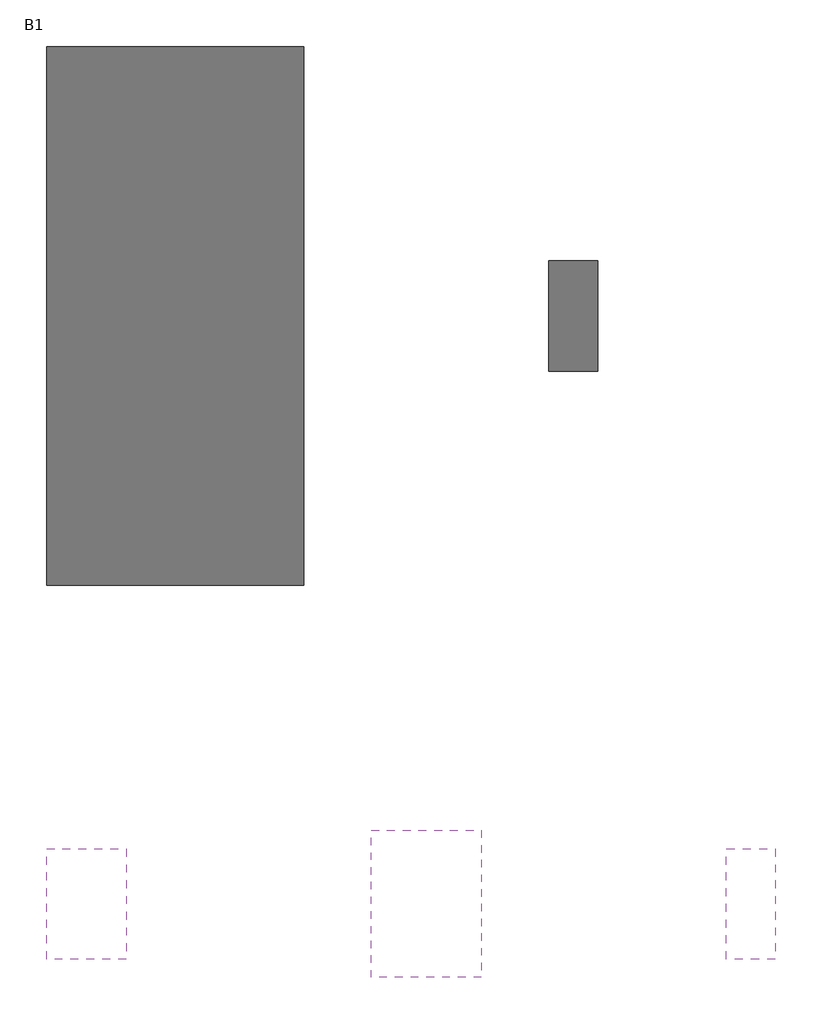
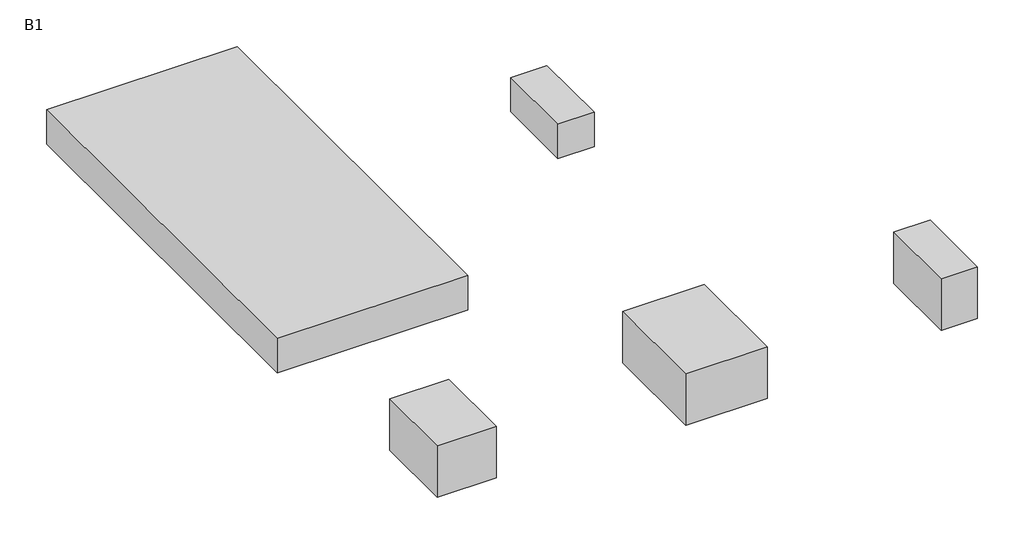
# One storey: 5 proxies.
"""IFC4 building model written with IfcOpenShell, lengths in millimetres."""

import ifcopenshell
import ifcopenshell.guid

model = None  # the IFC model being written
_history = None  # IfcOwnerHistory: only IFC2X3 demands one
_inside = {}  # id of a spatial element -> (the spatial element, [elements in it])
_under = {}  # id of a project, library or spatial element -> (it, [spatial elements below it])
_declared = {}  # id of a project -> (the project, [libraries it declares])
_typed = {}  # id of a type object -> (the type object, [elements of that type])
_made_of = {}  # id of a material, layer set ... -> (it, [elements and type objects made of it])


def new_model(schema):
    """Start an empty IFC model of exactly this schema.

    Asked for "IFC4X3", IfcOpenShell would pick the latest addendum, in which some entities
    have other attributes; the version numbers below select the first issue.
    IFC2X3 requires an IfcOwnerHistory on every rooted entity: one is made here for all.
    """
    global model, _history
    if schema == "IFC4X3":
        model = ifcopenshell.file(schema_version=(4, 3, 0, 0))
    else:
        model = ifcopenshell.file(schema=schema)
    _inside.clear()
    _under.clear()
    _declared.clear()
    _typed.clear()
    _made_of.clear()
    _history = None
    if model.schema == "IFC2X3":
        org = make("IfcOrganization", Name="unknown")
        user = make(
            "IfcPersonAndOrganization",
            ThePerson=make("IfcPerson", FamilyName="unknown"),
            TheOrganization=org,
        )
        app = make(
            "IfcApplication",
            ApplicationDeveloper=org,
            Version="unknown",
            ApplicationFullName="unknown",
            ApplicationIdentifier="unknown",
        )
        _history = make(
            "IfcOwnerHistory",
            OwningUser=user,
            OwningApplication=app,
            ChangeAction="ADDED",
            CreationDate=0,
        )
    return model


def make(cls, **values):
    """One entity of the class cls with the attributes given. An attribute that is None is left unset."""
    return model.create_entity(
        cls, **{name: value for name, value in values.items() if value is not None}
    )


def rooted(cls, **values):
    """An entity with a GlobalId (a new one), such as an element, a storey or a relation."""
    return make(cls, GlobalId=ifcopenshell.guid.new(), OwnerHistory=_history, **values)


def si_unit(unit_type, name, prefix=None):
    """IfcSIUnit, for example si_unit("LENGTHUNIT", "METRE", prefix="MILLI")."""
    return make("IfcSIUnit", UnitType=unit_type, Prefix=prefix, Name=name)


def assignment(units):
    """IfcUnitAssignment: the units of a project."""
    return None if units is None else make("IfcUnitAssignment", Units=units)


def point(xyz):
    """IfcCartesianPoint."""
    return None if xyz is None else make("IfcCartesianPoint", Coordinates=xyz)


def direction(xyz):
    """IfcDirection."""
    return None if xyz is None else make("IfcDirection", DirectionRatios=xyz)


def frame(location, z_axis=None, x_axis=None):
    """IfcAxis2Placement3D, a coordinate frame: its origin and axes. An axis left out is left unset."""
    return make(
        "IfcAxis2Placement3D",
        Location=point(location),
        Axis=direction(z_axis),
        RefDirection=direction(x_axis),
    )


def origin():
    """The frame at (0, 0, 0) with its axes left unset."""
    return frame((0.0, 0.0, 0.0))


def origin_with_axes():
    """The frame at (0, 0, 0) with the z axis (0, 0, 1) and the x axis (1, 0, 0) written out."""
    return frame((0.0, 0.0, 0.0), z_axis=(0.0, 0.0, 1.0), x_axis=(1.0, 0.0, 0.0))


def place(relative_to, where):
    """IfcLocalPlacement: puts the frame where relative to a parent placement (None: the world)."""
    return make(
        "IfcLocalPlacement", PlacementRelTo=relative_to, RelativePlacement=where
    )


def context(
    kind, dimensions, precision=None, world=None, true_north=None, identifier=None
):
    """IfcGeometricRepresentationContext, for example the 3D "Model" context."""
    return make(
        "IfcGeometricRepresentationContext",
        ContextIdentifier=identifier,
        ContextType=kind,
        CoordinateSpaceDimension=dimensions,
        Precision=precision,
        WorldCoordinateSystem=world,
        TrueNorth=true_north,
    )


def project(units=None, contexts=None):
    """IfcProject with its units and contexts."""
    return rooted(
        "IfcProject",
        Name="project",
        RepresentationContexts=contexts,
        UnitsInContext=assignment(units),
    )


def spatial(cls, under=None, at=None, **own):
    """A site, building, storey or space (cls), placed at a placement, below another one or the project."""
    s = rooted(cls, ObjectPlacement=at, **own)
    if under is not None:
        _under.setdefault(under.id(), (under, []))[1].append(s)
    return s


def polyline(points):
    """IfcPolyline through the points."""
    return make("IfcPolyline", Points=[point(p) for p in points])


def outline(outer, holes=None, kind="AREA"):
    """IfcArbitraryClosedProfileDef: a profile drawn as a closed curve; with holes, ...WithVoids."""
    if holes is None:
        return make("IfcArbitraryClosedProfileDef", ProfileType=kind, OuterCurve=outer)
    return make(
        "IfcArbitraryProfileDefWithVoids",
        ProfileType=kind,
        OuterCurve=outer,
        InnerCurves=holes,
    )


def extrude(swept, where, along, depth):
    """IfcExtrudedAreaSolid: the profile swept, set in the frame where, extruded along a direction by depth."""
    return make(
        "IfcExtrudedAreaSolid",
        SweptArea=swept,
        Position=where,
        ExtrudedDirection=direction(along),
        Depth=depth,
    )


def shape(context_of_items, identifier, shape_type, items):
    """IfcShapeRepresentation: the items that make up one representation, for example the "Body"."""
    return make(
        "IfcShapeRepresentation",
        ContextOfItems=context_of_items,
        RepresentationIdentifier=identifier,
        RepresentationType=shape_type,
        Items=items,
    )


def source(mapping_origin, context_of_items, identifier, shape_type, items):
    """IfcRepresentationMap: a shape defined once, which mapped items show again and again."""
    return make(
        "IfcRepresentationMap",
        MappingOrigin=mapping_origin,
        MappedRepresentation=shape(context_of_items, identifier, shape_type, items),
    )


def transform(
    local_origin,
    x_axis=None,
    y_axis=None,
    z_axis=None,
    scale=None,
    scale2=None,
    scale3=None,
    uniform=True,
):
    """IfcCartesianTransformationOperator3D, or its non-uniform kind. x_axis, y_axis, z_axis: its Axis1, 2, 3."""
    if uniform:
        return make(
            "IfcCartesianTransformationOperator3D",
            Axis1=direction(x_axis),
            Axis2=direction(y_axis),
            LocalOrigin=point(local_origin),
            Scale=scale,
            Axis3=direction(z_axis),
        )
    return make(
        "IfcCartesianTransformationOperator3DnonUniform",
        Axis1=direction(x_axis),
        Axis2=direction(y_axis),
        LocalOrigin=point(local_origin),
        Scale=scale,
        Axis3=direction(z_axis),
        Scale2=scale2,
        Scale3=scale3,
    )


def mapped(mapping_source, mapping_target):
    """IfcMappedItem: shows the shape of a source again, moved by a transform."""
    return make(
        "IfcMappedItem", MappingSource=mapping_source, MappingTarget=mapping_target
    )


def made_of(thing, what):
    """Note that an element or type object is made of a material, layer set ...; save() writes the relation."""
    if what is not None:
        _made_of.setdefault(what.id(), (what, []))[1].append(thing)
    return thing


def element(
    cls,
    number,
    at=None,
    inside=None,
    cuts=None,
    type_object=None,
    material=None,
    context=None,
    identifier="Body",
    shape_type=None,
    held_by="IfcProductDefinitionShape",
    body=None,
    shapes=None,
    **own,
):
    """One element of the class cls, such as IfcWall. Its Tag is "e" and its number.

    at: its placement. inside: the storey or other place that contains it. cuts: it is an
    opening in that element (IfcRelVoidsElement). A single representation is given by context,
    identifier, shape_type and body (its items); several are given by shapes. held_by: the class
    of the entity that holds the representations. save() writes the other relations.
    """
    e = rooted(cls, Tag="e%d" % number, ObjectPlacement=at, **own)
    if body is not None:
        shapes = [shape(context, identifier, shape_type, body)]
    if shapes is not None:
        e.Representation = make(held_by, Representations=shapes)
    if inside is not None:
        _inside.setdefault(inside.id(), (inside, []))[1].append(e)
    if cuts is not None:
        rooted(
            "IfcRelVoidsElement", RelatingBuildingElement=cuts, RelatedOpeningElement=e
        )
    if type_object is not None:
        _typed.setdefault(type_object.id(), (type_object, []))[1].append(e)
    return made_of(e, material)


def aggregate(whole, parts):
    """IfcRelAggregates: a whole, such as a stair, and the parts it consists of."""
    return rooted("IfcRelAggregates", RelatingObject=whole, RelatedObjects=parts)


def save(model, path):
    """Write the relations noted so far, then the file.

    IfcRelAggregates (storeys below a building ...), IfcRelContainedInSpatialStructure (elements
    in a storey), IfcRelDefinesByType, IfcRelAssociatesMaterial and IfcRelDeclares: one each for
    every whole, place, type object, material and project.
    """
    for whole, parts in _under.values():
        aggregate(whole, parts)
    for where, things in _inside.values():
        rooted(
            "IfcRelContainedInSpatialStructure",
            RelatedElements=things,
            RelatingStructure=where,
        )
    for kind, things in _typed.values():
        rooted("IfcRelDefinesByType", RelatedObjects=things, RelatingType=kind)
    for what, things in _made_of.values():
        rooted("IfcRelAssociatesMaterial", RelatedObjects=things, RelatingMaterial=what)
    for by, libraries in _declared.values():
        rooted("IfcRelDeclares", RelatingContext=by, RelatedDefinitions=libraries)
    model.write(path)


def generic_models_1d705098(model_context):
    return source(origin(), model_context, "Body", "SweptSolid", [
        extrude(outline(polyline([(3250.0, 4500.0), (3250.0, -4500.0), (-3250.0, -4500.0), (-3250.0, 4500.0), (3250.0, 4500.0)])), origin_with_axes(), (0.0, 0.0, 1.0), 6000.0),
    ])


def generic_models_399a6151(model_context):
    return source(origin(), model_context, "Body", "SweptSolid", [
        extrude(outline(polyline([(4500.0, 6000.0), (4500.0, -6000.0), (-4500.0, -6000.0), (-4500.0, 6000.0), (4500.0, 6000.0)])), origin_with_axes(), (0.0, 0.0, 1.0), 6000.0),
    ])


def generic_models_29bcd6f9(model_context):
    return source(origin(), model_context, "Body", "SweptSolid", [
        extrude(outline(polyline([(2000.0, 4500.0), (2000.0, -4500.0), (-2000.0, -4500.0), (-2000.0, 4500.0), (2000.0, 4500.0)])), origin_with_axes(), (0.0, 0.0, 1.0), 6000.0),
    ])


def generic_models_a454a2aa(model_context):
    return source(origin(), model_context, "Body", "SweptSolid", [
        extrude(outline(polyline([(10500.0, 22000.0), (10500.0, -22000.0), (-10500.0, -22000.0), (-10500.0, 22000.0), (10500.0, 22000.0)])), origin_with_axes(), (0.0, 0.0, 1.0), 4000.0),
    ])


def generic_models_73802227(model_context):
    return source(origin(), model_context, "Body", "SweptSolid", [
        extrude(outline(polyline([(2000.0, 4500.0), (2000.0, -4500.0), (-2000.0, -4500.0), (-2000.0, 4500.0), (2000.0, 4500.0)])), origin_with_axes(), (0.0, 0.0, 1.0), 4000.0),
    ])


model = new_model("IFC4")

# Units and contexts
model_context = context("Model", 3, world=origin())
ifc_project = project(units=[si_unit("LENGTHUNIT", "METRE", prefix="MILLI")], contexts=[model_context])

# Site, building, storey
site = spatial("IfcSite", under=ifc_project)
building = spatial("IfcBuilding", under=site)
storey = spatial("IfcBuildingStorey", under=building, Name="B1", Elevation=-4000.0)

# Proxies
placement = place(None, origin())
generic_models_shape = generic_models_1d705098(model_context)
element("IfcBuildingElementProxy", 1, Name="Space Planning Box_hec : Space Planning Box_hec", ObjectType="Space Planning Box_hec : Space Planning Box_hec", at=placement, inside=storey, context=model_context, shape_type="MappedRepresentation", body=[
    mapped(generic_models_shape, transform((3250.0, 6000.0, 0.0), x_axis=(1.0, 0.0, 0.0), y_axis=(0.0, 1.0, 0.0), z_axis=(0.0, 0.0, 1.0))),
])
generic_models_2_shape = generic_models_399a6151(model_context)
element("IfcBuildingElementProxy", 2, Name="Space Planning Box_hec : Space Planning Box_hec", ObjectType="Space Planning Box_hec : Space Planning Box_hec", at=placement, inside=storey, context=model_context, shape_type="MappedRepresentation", body=[
    mapped(generic_models_2_shape, transform((31000.0, 6000.0, 0.0), x_axis=(1.0, 0.0, 0.0), y_axis=(0.0, 1.0, 0.0), z_axis=(0.0, 0.0, 1.0))),
])
generic_models_3_shape = generic_models_29bcd6f9(model_context)
element("IfcBuildingElementProxy", 3, Name="Space Planning Box_hec : Space Planning Box_hec", ObjectType="Space Planning Box_hec : Space Planning Box_hec", at=placement, inside=storey, context=model_context, shape_type="MappedRepresentation", body=[
    mapped(generic_models_3_shape, transform((57500.0, 6000.0, 0.0), x_axis=(1.0, 0.0, 0.0), y_axis=(0.0, 1.0, 0.0), z_axis=(0.0, 0.0, 1.0))),
])
generic_models_4_shape = generic_models_a454a2aa(model_context)
element("IfcBuildingElementProxy", 4, Name="Space Planning Box_hec : Space Planning Box_hec", ObjectType="Space Planning Box_hec : Space Planning Box_hec", at=placement, inside=storey, context=model_context, shape_type="MappedRepresentation", body=[
    mapped(generic_models_4_shape, transform((10500.0, 54000.0, -4000.0), x_axis=(1.0, 0.0, 0.0), y_axis=(0.0, 1.0, 0.0), z_axis=(0.0, 0.0, 1.0))),
])
generic_models_5_shape = generic_models_73802227(model_context)
element("IfcBuildingElementProxy", 5, Name="Space Planning Box_hec : Space Planning Box_hec", ObjectType="Space Planning Box_hec : Space Planning Box_hec", at=placement, inside=storey, context=model_context, shape_type="MappedRepresentation", body=[
    mapped(generic_models_5_shape, transform((43000.0, 54000.0, -4000.0), x_axis=(1.0, 0.0, 0.0), y_axis=(0.0, 1.0, 0.0), z_axis=(0.0, 0.0, 1.0))),
])

save(model, "model.ifc")

# Revit data of these elements
# Project information
#   Building Name = "MAIN GATE SECURITY BUILDING"
#   Project Status = "Project Status"
#   Client Name = "현대엔지니어링"
#   Project Address = "서울시 종로구 율곡로 75(계동)"
#   Project Name = "Therma Visayas Energy Project"
#   Project Number = "-"
# Grids (mm)
#   "A": line (45459.652, 190234.526) -> (45459.652, 152139.384)
#   "B": line (53459.652, 190234.526) -> (53459.652, 152139.384)
#   "C": line (61459.652, 190234.526) -> (61459.652, 152139.384)
#   "D": line (67459.652, 190234.526) -> (67459.652, 152139.384)
#   "E": line (73459.652, 190234.526) -> (73459.652, 152139.384)
#   "F": line (81459.652, 190234.526) -> (81459.652, 152139.384)
#   "G": line (85459.652, 190234.526) -> (85459.652, 152139.384)
#   "H": line (89459.652, 190234.526) -> (89459.652, 152139.384)
#   "4": line (39389.066, 184923.861) -> (102402.798, 184923.861)
#   "3": line (39389.066, 178923.861) -> (102402.798, 178923.861)
#   "2": line (39389.066, 172923.861) -> (102402.798, 172923.861)
#   "1": line (39389.066, 163923.861) -> (102402.798, 163923.861)
# Type "Space Planning Box_hec : Space Planning Box_hec"
#   Type Comments = "..."
#   Room Name [instance default] = "?"
#   Interior Finish [instance default] = ""
#   Exterior Finish [instance default] = ""
#   Department [instance default] = ""
#   Assembly Code = "..."
#   Width [instance default] = 1524 mm
#   Program Area [instance default] = 0.00 m²
#   Length [instance default] = 1524 mm
#   Height [instance default] = 1524 mm
#   Area [instance default] = 2.32258 m²
#   Fill Color [instance default] = Cyan
#   Default Elevation = 0
# Element 1 (IfcBuildingElementProxy, "Space Planning Box_hec : Space Planning Box_hec")
#   Room Name = "Switchgear Room"
#   Interior Finish = "IF1"
#   Exterior Finish = "EF1"
#   Department = "EL"
#   Width = 6500 mm
#   Program Area = 58.50 m²
#   Length = 9000 mm
#   Height = 6000 mm
#   Area = 58.50 m²
#   Fill Color = Blue
#   Phase Created = New Construction
#   Materials on its faces: "Blue"
# Element 2 (IfcBuildingElementProxy, "Space Planning Box_hec : Space Planning Box_hec")
#   Room Name = "Battery Room"
#   Interior Finish = "IF4"
#   Exterior Finish = "EF1"
#   Department = "EL"
#   Width = 9000 mm
#   Program Area = 108.00 m²
#   Length = 12000 mm
#   Height = 6000 mm
#   Area = 108.00 m²
#   Fill Color = Blue
#   Phase Created = New Construction
#   Materials on its faces: "Blue"
# Element 3 (IfcBuildingElementProxy, "Space Planning Box_hec : Space Planning Box_hec")
#   Room Name = "Stairway"
#   Interior Finish = "IF2"
#   Exterior Finish = "EF1"
#   Department = "AR"
#   Width = 4000 mm
#   Program Area = 36.00 m²
#   Length = 9000 mm
#   Height = 6000 mm
#   Area = 36.00 m²
#   Fill Color = Lavender
#   Phase Created = New Construction
#   Materials on its faces: "Lavender"
# Element 4 (IfcBuildingElementProxy, "Space Planning Box_hec : Space Planning Box_hec")
#   Room Name = "Cable Room"
#   Interior Finish = "IF1"
#   Exterior Finish = "EF1"
#   Department = "EL"
#   Width = 21000 mm
#   Program Area = 924.00 m²
#   Length = 44000 mm
#   Height = 4000 mm
#   Area = 924.00 m²
#   Fill Color = Blue
#   Phase Created = New Construction
#   Materials on its faces: "Blue"
# Element 5 (IfcBuildingElementProxy, "Space Planning Box_hec : Space Planning Box_hec")
#   Room Name = "Stairway"
#   Interior Finish = "IF2"
#   Exterior Finish = "EF1"
#   Department = "EL"
#   Width = 4000 mm
#   Program Area = 36.00 m²
#   Length = 9000 mm
#   Height = 4000 mm
#   Area = 36.00 m²
#   Fill Color = Blue
#   Phase Created = New Construction
#   Materials on its faces: "Blue"
# Materials
#   "Cyan": class "Generic", colour RGB 0 255 255, transparency 0.2, Cost = 0
#   "Blue": class "Generic", colour RGB 0 0 255, transparency 0.2, Cost = 0
#   "Lavender": class "Generic", colour RGB 186 85 211, transparency 0.2, Cost = 0
